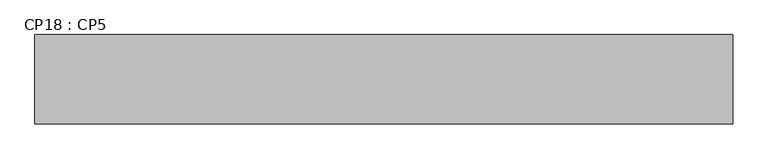
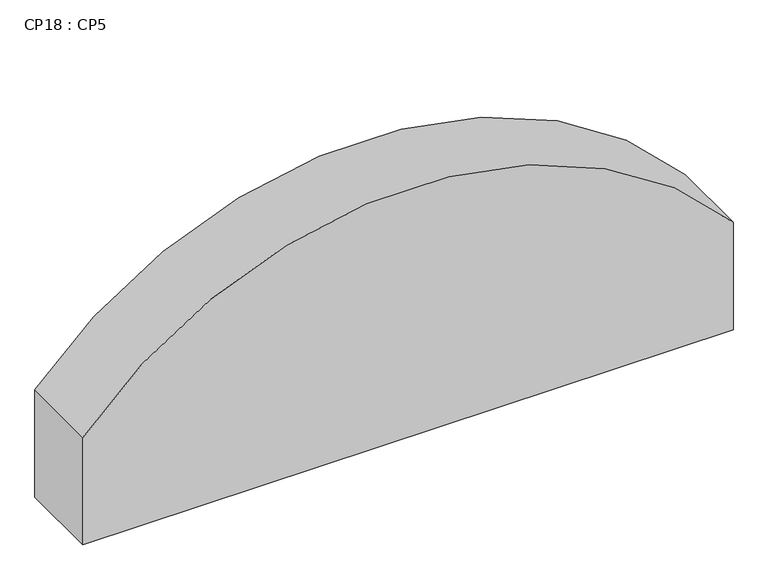
"""IFC4 building model written with IfcOpenShell, lengths in millimetres: beam geometry, CP18 : CP5."""

from ifc_helpers import new_model, si_unit, frame, origin, place, context, project, spatial, circle_curve, source, transform, mapped, element, save
from ifc_brep_helpers import plane_surface, cylinder_surface, advanced_brep


def cp18_cp5_e7e1a95e(model_context):
    return source(origin(), model_context, "Body", "AdvancedBrep", [
        advanced_brep(
        [(4843.2245516, 20099.7448193, 14620.0), (4843.2245516, 20099.7448193, 13800.0), (143.2245521, 20099.7448193, 13800.0), (143.2245521, 20099.7448193, 14620.0), (4843.2245542, 19499.6999972, 14620.0), (143.2245543, 19499.6999972, 14620.0), (143.2245521, 19499.6999972, 13800.0), (4843.2245516, 19499.6999972, 13800.0)],
        [
            (0, 1),
            (1, 2),
            (2, 3),
            (3, 0, circle_curve(frame((2493.2245543, 20099.7448193, 12608.2612414), z_axis=(0.0, 1.0, 0.0), x_axis=(0.0, 0.0, -1.0)), 3093.4758497)),
            (4, 5, circle_curve(frame((2493.2245543, 19499.6999972, 12608.2612414), z_axis=(0.0, -1.0, 0.0), x_axis=(0.0, 0.0, -1.0)), 3093.4758497)),
            (5, 6),
            (6, 7),
            (7, 4),
            (1, 7),
            (6, 2),
            (4, 0),
            (3, 5),
        ],
        [
            plane_surface(frame((2418.2245543, 20099.7448193, 9004.7654345), z_axis=(0.0, 1.0, 0.0), x_axis=(-1.0, 0.0, 0.0))),
            plane_surface(frame((2418.2245543, 19499.6999972, 9004.7654345), z_axis=(0.0, -1.0, 0.0), x_axis=(1.0, 0.0, 0.0))),
            plane_surface(frame((4993.2245542, 20099.7448193, 13800.0), z_axis=(0.0, 0.0, -1.0), x_axis=(0.0, -1.0, 0.0))),
            cylinder_surface(frame((2493.2245543, 20099.7448193, 12608.2612414), z_axis=(0.0, 1.0, 0.0), x_axis=(0.0, 0.0, -1.0)), 3093.4758497),
            plane_surface(frame((4843.2245516, 18587.0448193, 13800.0), z_axis=(1.0, 0.0, 0.0), x_axis=(0.0, -1.0, 0.0))),
            plane_surface(frame((143.2245521, 18587.0448193, 14620.0), z_axis=(-1.0, 0.0, 0.0), x_axis=(0.0, -1.0, 0.0))),
        ],
        [
            (0, [[1, 2, 3, 4]]),
            (1, [[5, 6, 7, 8]]),
            (2, [[9, -7, 10, -2]]),
            (3, [[-5, 11, -4, 12]]),
            (4, [[-1, -11, -8, -9]]),
            (5, [[-3, -10, -6, -12]]),
        ],
    ),
    ])


if __name__ == "__main__":
    model = new_model("IFC4")
    model_context = context("Model", 3, world=origin())
    ifc_project = project(units=[si_unit("LENGTHUNIT", "METRE", prefix="MILLI")], contexts=[model_context])
    site = spatial("IfcSite", under=ifc_project)
    building = spatial("IfcBuilding", under=site)
    placement = place(None, origin())
    cp18_cp5_shape = cp18_cp5_e7e1a95e(model_context)
    element("IfcBeam", 1, ObjectType="CP18 : CP5", at=placement, inside=building, context=model_context, shape_type="MappedRepresentation", body=[
        mapped(cp18_cp5_shape, transform((0.0, 0.0, 0.0), x_axis=(1.0, 0.0, 0.0), y_axis=(0.0, 1.0, 0.0), z_axis=(0.0, 0.0, 1.0))),
    ])
    save(model, "model.ifc")
